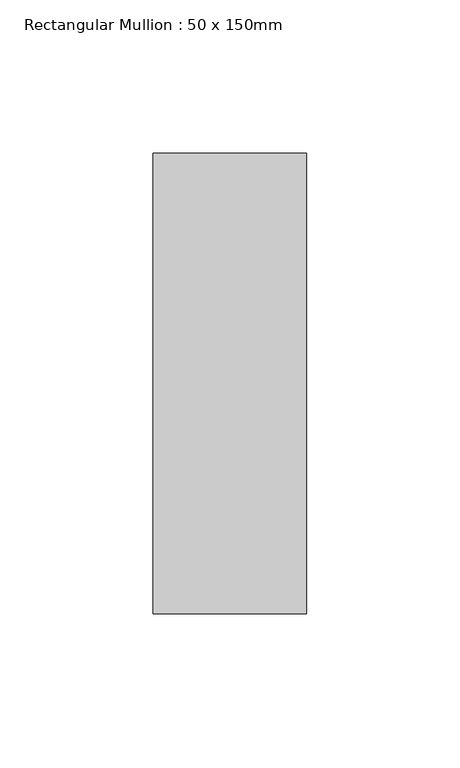
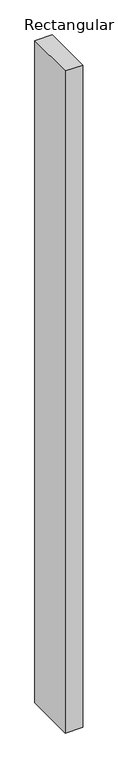
"""IFC4 building model written with IfcOpenShell, lengths in millimetres: member geometry, Rectangular Mullion : 50 x 150mm."""

import ifcopenshell
import ifcopenshell.guid

model = None  # the IFC model being written
_history = None  # IfcOwnerHistory: only IFC2X3 demands one
_inside = {}  # id of a spatial element -> (the spatial element, [elements in it])
_under = {}  # id of a project, library or spatial element -> (it, [spatial elements below it])
_declared = {}  # id of a project -> (the project, [libraries it declares])
_typed = {}  # id of a type object -> (the type object, [elements of that type])
_made_of = {}  # id of a material, layer set ... -> (it, [elements and type objects made of it])


def new_model(schema):
    """Start an empty IFC model of exactly this schema.

    Asked for "IFC4X3", IfcOpenShell would pick the latest addendum, in which some entities
    have other attributes; the version numbers below select the first issue.
    IFC2X3 requires an IfcOwnerHistory on every rooted entity: one is made here for all.
    """
    global model, _history
    if schema == "IFC4X3":
        model = ifcopenshell.file(schema_version=(4, 3, 0, 0))
    else:
        model = ifcopenshell.file(schema=schema)
    _inside.clear()
    _under.clear()
    _declared.clear()
    _typed.clear()
    _made_of.clear()
    _history = None
    if model.schema == "IFC2X3":
        org = make("IfcOrganization", Name="unknown")
        user = make(
            "IfcPersonAndOrganization",
            ThePerson=make("IfcPerson", FamilyName="unknown"),
            TheOrganization=org,
        )
        app = make(
            "IfcApplication",
            ApplicationDeveloper=org,
            Version="unknown",
            ApplicationFullName="unknown",
            ApplicationIdentifier="unknown",
        )
        _history = make(
            "IfcOwnerHistory",
            OwningUser=user,
            OwningApplication=app,
            ChangeAction="ADDED",
            CreationDate=0,
        )
    return model


def make(cls, **values):
    """One entity of the class cls with the attributes given. An attribute that is None is left unset."""
    return model.create_entity(
        cls, **{name: value for name, value in values.items() if value is not None}
    )


def rooted(cls, **values):
    """An entity with a GlobalId (a new one), such as an element, a storey or a relation."""
    return make(cls, GlobalId=ifcopenshell.guid.new(), OwnerHistory=_history, **values)


def si_unit(unit_type, name, prefix=None):
    """IfcSIUnit, for example si_unit("LENGTHUNIT", "METRE", prefix="MILLI")."""
    return make("IfcSIUnit", UnitType=unit_type, Prefix=prefix, Name=name)


def assignment(units):
    """IfcUnitAssignment: the units of a project."""
    return None if units is None else make("IfcUnitAssignment", Units=units)


def point(xyz):
    """IfcCartesianPoint."""
    return None if xyz is None else make("IfcCartesianPoint", Coordinates=xyz)


def direction(xyz):
    """IfcDirection."""
    return None if xyz is None else make("IfcDirection", DirectionRatios=xyz)


def frame(location, z_axis=None, x_axis=None):
    """IfcAxis2Placement3D, a coordinate frame: its origin and axes. An axis left out is left unset."""
    return make(
        "IfcAxis2Placement3D",
        Location=point(location),
        Axis=direction(z_axis),
        RefDirection=direction(x_axis),
    )


def origin():
    """The frame at (0, 0, 0) with its axes left unset."""
    return frame((0.0, 0.0, 0.0))


def place(relative_to, where):
    """IfcLocalPlacement: puts the frame where relative to a parent placement (None: the world)."""
    return make(
        "IfcLocalPlacement", PlacementRelTo=relative_to, RelativePlacement=where
    )


def context(
    kind, dimensions, precision=None, world=None, true_north=None, identifier=None
):
    """IfcGeometricRepresentationContext, for example the 3D "Model" context."""
    return make(
        "IfcGeometricRepresentationContext",
        ContextIdentifier=identifier,
        ContextType=kind,
        CoordinateSpaceDimension=dimensions,
        Precision=precision,
        WorldCoordinateSystem=world,
        TrueNorth=true_north,
    )


def project(units=None, contexts=None):
    """IfcProject with its units and contexts."""
    return rooted(
        "IfcProject",
        Name="project",
        RepresentationContexts=contexts,
        UnitsInContext=assignment(units),
    )


def spatial(cls, under=None, at=None, **own):
    """A site, building, storey or space (cls), placed at a placement, below another one or the project."""
    s = rooted(cls, ObjectPlacement=at, **own)
    if under is not None:
        _under.setdefault(under.id(), (under, []))[1].append(s)
    return s


def polyline(points):
    """IfcPolyline through the points."""
    return make("IfcPolyline", Points=[point(p) for p in points])


def outline(outer, holes=None, kind="AREA"):
    """IfcArbitraryClosedProfileDef: a profile drawn as a closed curve; with holes, ...WithVoids."""
    if holes is None:
        return make("IfcArbitraryClosedProfileDef", ProfileType=kind, OuterCurve=outer)
    return make(
        "IfcArbitraryProfileDefWithVoids",
        ProfileType=kind,
        OuterCurve=outer,
        InnerCurves=holes,
    )


def extrude(swept, where, along, depth):
    """IfcExtrudedAreaSolid: the profile swept, set in the frame where, extruded along a direction by depth."""
    return make(
        "IfcExtrudedAreaSolid",
        SweptArea=swept,
        Position=where,
        ExtrudedDirection=direction(along),
        Depth=depth,
    )


def shape(context_of_items, identifier, shape_type, items):
    """IfcShapeRepresentation: the items that make up one representation, for example the "Body"."""
    return make(
        "IfcShapeRepresentation",
        ContextOfItems=context_of_items,
        RepresentationIdentifier=identifier,
        RepresentationType=shape_type,
        Items=items,
    )


def source(mapping_origin, context_of_items, identifier, shape_type, items):
    """IfcRepresentationMap: a shape defined once, which mapped items show again and again."""
    return make(
        "IfcRepresentationMap",
        MappingOrigin=mapping_origin,
        MappedRepresentation=shape(context_of_items, identifier, shape_type, items),
    )


def transform(
    local_origin,
    x_axis=None,
    y_axis=None,
    z_axis=None,
    scale=None,
    scale2=None,
    scale3=None,
    uniform=True,
):
    """IfcCartesianTransformationOperator3D, or its non-uniform kind. x_axis, y_axis, z_axis: its Axis1, 2, 3."""
    if uniform:
        return make(
            "IfcCartesianTransformationOperator3D",
            Axis1=direction(x_axis),
            Axis2=direction(y_axis),
            LocalOrigin=point(local_origin),
            Scale=scale,
            Axis3=direction(z_axis),
        )
    return make(
        "IfcCartesianTransformationOperator3DnonUniform",
        Axis1=direction(x_axis),
        Axis2=direction(y_axis),
        LocalOrigin=point(local_origin),
        Scale=scale,
        Axis3=direction(z_axis),
        Scale2=scale2,
        Scale3=scale3,
    )


def mapped(mapping_source, mapping_target):
    """IfcMappedItem: shows the shape of a source again, moved by a transform."""
    return make(
        "IfcMappedItem", MappingSource=mapping_source, MappingTarget=mapping_target
    )


def made_of(thing, what):
    """Note that an element or type object is made of a material, layer set ...; save() writes the relation."""
    if what is not None:
        _made_of.setdefault(what.id(), (what, []))[1].append(thing)
    return thing


def element(
    cls,
    number,
    at=None,
    inside=None,
    cuts=None,
    type_object=None,
    material=None,
    context=None,
    identifier="Body",
    shape_type=None,
    held_by="IfcProductDefinitionShape",
    body=None,
    shapes=None,
    **own,
):
    """One element of the class cls, such as IfcWall. Its Tag is "e" and its number.

    at: its placement. inside: the storey or other place that contains it. cuts: it is an
    opening in that element (IfcRelVoidsElement). A single representation is given by context,
    identifier, shape_type and body (its items); several are given by shapes. held_by: the class
    of the entity that holds the representations. save() writes the other relations.
    """
    e = rooted(cls, Tag="e%d" % number, ObjectPlacement=at, **own)
    if body is not None:
        shapes = [shape(context, identifier, shape_type, body)]
    if shapes is not None:
        e.Representation = make(held_by, Representations=shapes)
    if inside is not None:
        _inside.setdefault(inside.id(), (inside, []))[1].append(e)
    if cuts is not None:
        rooted(
            "IfcRelVoidsElement", RelatingBuildingElement=cuts, RelatedOpeningElement=e
        )
    if type_object is not None:
        _typed.setdefault(type_object.id(), (type_object, []))[1].append(e)
    return made_of(e, material)


def aggregate(whole, parts):
    """IfcRelAggregates: a whole, such as a stair, and the parts it consists of."""
    return rooted("IfcRelAggregates", RelatingObject=whole, RelatedObjects=parts)


def save(model, path):
    """Write the relations noted so far, then the file.

    IfcRelAggregates (storeys below a building ...), IfcRelContainedInSpatialStructure (elements
    in a storey), IfcRelDefinesByType, IfcRelAssociatesMaterial and IfcRelDeclares: one each for
    every whole, place, type object, material and project.
    """
    for whole, parts in _under.values():
        aggregate(whole, parts)
    for where, things in _inside.values():
        rooted(
            "IfcRelContainedInSpatialStructure",
            RelatedElements=things,
            RelatingStructure=where,
        )
    for kind, things in _typed.values():
        rooted("IfcRelDefinesByType", RelatedObjects=things, RelatingType=kind)
    for what, things in _made_of.values():
        rooted("IfcRelAssociatesMaterial", RelatedObjects=things, RelatingMaterial=what)
    for by, libraries in _declared.values():
        rooted("IfcRelDeclares", RelatingContext=by, RelatedDefinitions=libraries)
    model.write(path)


def rectangular_mullion_50_x_150mm_aa47fe12(model_context):
    return source(origin(), model_context, "Body", "SweptSolid", [
        extrude(outline(polyline([(0.0, 75.0), (0.0, -75.0), (-50.0, -75.0), (-50.0, 75.0), (0.0, 75.0)])), frame((0.0, 0.0, -2000.0), z_axis=(0.0, 0.0, 1.0), x_axis=(1.0, 0.0, 0.0)), (0.0, 0.0, 1.0), 2000.0),
    ])


if __name__ == "__main__":
    model = new_model("IFC4")
    model_context = context("Model", 3, world=origin())
    ifc_project = project(units=[si_unit("LENGTHUNIT", "METRE", prefix="MILLI")], contexts=[model_context])
    site = spatial("IfcSite", under=ifc_project)
    building = spatial("IfcBuilding", under=site)
    placement = place(None, origin())
    rectangular_mullion_50_x_150mm_shape = rectangular_mullion_50_x_150mm_aa47fe12(model_context)
    element("IfcMember", 1, ObjectType="Rectangular Mullion : 50 x 150mm", at=placement, inside=building, context=model_context, shape_type="MappedRepresentation", body=[
        mapped(rectangular_mullion_50_x_150mm_shape, transform((0.0, 0.0, 0.0), x_axis=(1.0, 0.0, 0.0), y_axis=(0.0, 1.0, 0.0), z_axis=(0.0, 0.0, 1.0))),
    ])
    save(model, "model.ifc")

# Revit data of these elements
# Type "Rectangular Mullion : 50 x 150mm"
#   built-in parameter 1007304 = 0.492126 (stored number, unit not read)
#   built-in parameter 1007301 = 0.082021 (stored number, unit not read)
#   built-in parameter 1007300 = 0.082021 (stored number, unit not read)
# Element 1 (IfcMember, "Rectangular Mullion : 50 x 150mm")
#   Materials on its faces: "Metal - Aluminium"
# Materials
#   "Metal - Aluminium": class "Metal", colour RGB 247 247 247, transparency 0
